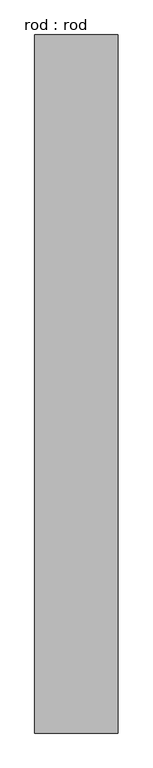
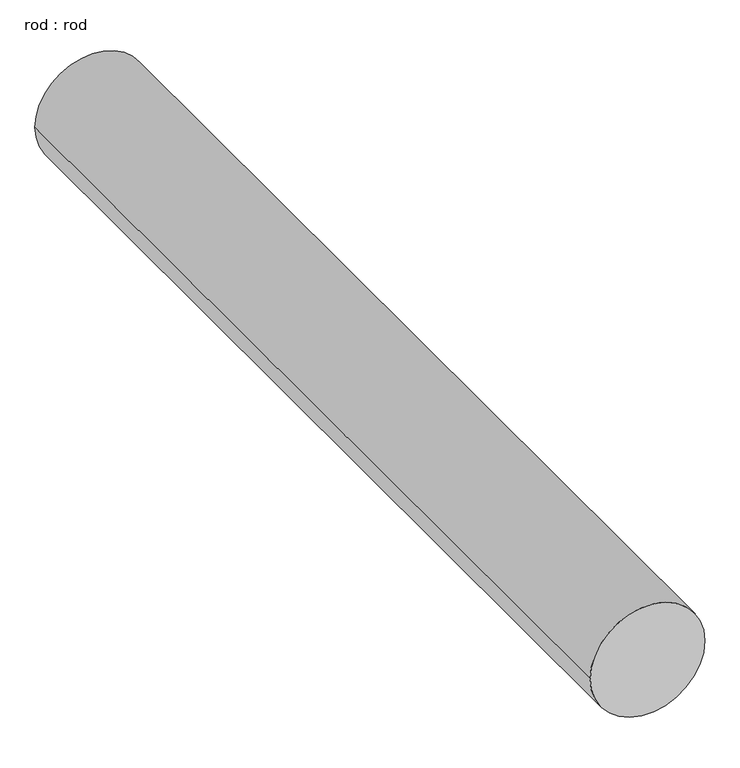
"""IFC4 building model written with IfcOpenShell, lengths in millimetres: proxy geometry, rod : rod."""

from ifc_helpers import new_model, si_unit, point, frame, frame_2d, origin, place, context, project, spatial, circle_curve, trimmed, segment, composite_curve, outline, extrude, source, transform, mapped, element, save


def rod_rod_b0048661(model_context):
    return source(origin(), model_context, "Body", "SweptSolid", [
        extrude(outline(composite_curve([segment(trimmed(circle_curve(frame_2d((0.0108462, 0.0)), 200.0), [point((0.0108462, 200.0))], [point((0.0108462, -200.0))], False, "CARTESIAN"), True, "CONTINUOUS"), segment(trimmed(circle_curve(frame_2d((0.0108462, 0.0)), 200.0), [point((0.0108462, -200.0))], [point((0.0108462, 200.0))], False, "CARTESIAN"), True, "CONTINUOUS")], self_intersect=False)), frame((0.0, 2415.9429011, 0.0), z_axis=(0.0, 1.0, 0.0), x_axis=(0.0, 0.0, 1.0)), (0.0, 0.0, 1.0), 3353.5714286),
    ])


if __name__ == "__main__":
    model = new_model("IFC4")
    model_context = context("Model", 3, world=origin())
    ifc_project = project(units=[si_unit("LENGTHUNIT", "METRE", prefix="MILLI")], contexts=[model_context])
    site = spatial("IfcSite", under=ifc_project)
    building = spatial("IfcBuilding", under=site)
    placement = place(None, origin())
    rod_rod_shape = rod_rod_b0048661(model_context)
    element("IfcBuildingElementProxy", 1, Name="rod : rod", ObjectType="rod : rod", at=placement, inside=building, context=model_context, shape_type="MappedRepresentation", body=[
        mapped(rod_rod_shape, transform((0.0, 0.0, 0.0), x_axis=(1.0, 0.0, 0.0), y_axis=(0.0, 1.0, 0.0), z_axis=(0.0, 0.0, 1.0))),
    ])
    save(model, "model.ifc")

# Revit data of these elements
# Type "rod : rod"
#   Default Elevation = 0
